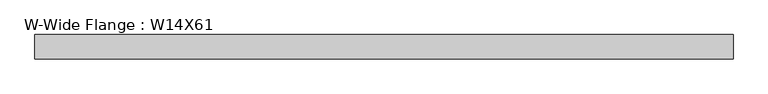
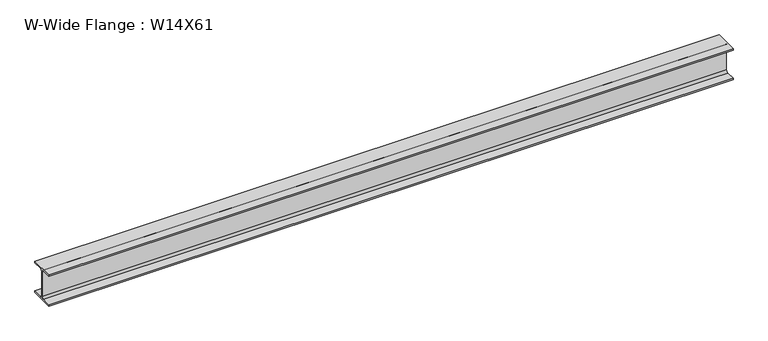
"""IFC4 building model written with IfcOpenShell, lengths in millimetres: beam geometry, W-Wide Flange : W14X61."""

import ifcopenshell
import ifcopenshell.guid

model = None  # the IFC model being written
_history = None  # IfcOwnerHistory: only IFC2X3 demands one
_inside = {}  # id of a spatial element -> (the spatial element, [elements in it])
_under = {}  # id of a project, library or spatial element -> (it, [spatial elements below it])
_declared = {}  # id of a project -> (the project, [libraries it declares])
_typed = {}  # id of a type object -> (the type object, [elements of that type])
_made_of = {}  # id of a material, layer set ... -> (it, [elements and type objects made of it])


def new_model(schema):
    """Start an empty IFC model of exactly this schema.

    Asked for "IFC4X3", IfcOpenShell would pick the latest addendum, in which some entities
    have other attributes; the version numbers below select the first issue.
    IFC2X3 requires an IfcOwnerHistory on every rooted entity: one is made here for all.
    """
    global model, _history
    if schema == "IFC4X3":
        model = ifcopenshell.file(schema_version=(4, 3, 0, 0))
    else:
        model = ifcopenshell.file(schema=schema)
    _inside.clear()
    _under.clear()
    _declared.clear()
    _typed.clear()
    _made_of.clear()
    _history = None
    if model.schema == "IFC2X3":
        org = make("IfcOrganization", Name="unknown")
        user = make(
            "IfcPersonAndOrganization",
            ThePerson=make("IfcPerson", FamilyName="unknown"),
            TheOrganization=org,
        )
        app = make(
            "IfcApplication",
            ApplicationDeveloper=org,
            Version="unknown",
            ApplicationFullName="unknown",
            ApplicationIdentifier="unknown",
        )
        _history = make(
            "IfcOwnerHistory",
            OwningUser=user,
            OwningApplication=app,
            ChangeAction="ADDED",
            CreationDate=0,
        )
    return model


def make(cls, **values):
    """One entity of the class cls with the attributes given. An attribute that is None is left unset."""
    return model.create_entity(
        cls, **{name: value for name, value in values.items() if value is not None}
    )


def rooted(cls, **values):
    """An entity with a GlobalId (a new one), such as an element, a storey or a relation."""
    return make(cls, GlobalId=ifcopenshell.guid.new(), OwnerHistory=_history, **values)


def si_unit(unit_type, name, prefix=None):
    """IfcSIUnit, for example si_unit("LENGTHUNIT", "METRE", prefix="MILLI")."""
    return make("IfcSIUnit", UnitType=unit_type, Prefix=prefix, Name=name)


def assignment(units):
    """IfcUnitAssignment: the units of a project."""
    return None if units is None else make("IfcUnitAssignment", Units=units)


def point(xyz):
    """IfcCartesianPoint."""
    return None if xyz is None else make("IfcCartesianPoint", Coordinates=xyz)


def direction(xyz):
    """IfcDirection."""
    return None if xyz is None else make("IfcDirection", DirectionRatios=xyz)


def frame(location, z_axis=None, x_axis=None):
    """IfcAxis2Placement3D, a coordinate frame: its origin and axes. An axis left out is left unset."""
    return make(
        "IfcAxis2Placement3D",
        Location=point(location),
        Axis=direction(z_axis),
        RefDirection=direction(x_axis),
    )


def frame_2d(location, x_axis=None):
    """IfcAxis2Placement2D, a coordinate frame in the plane: its origin and x axis."""
    return make(
        "IfcAxis2Placement2D", Location=point(location), RefDirection=direction(x_axis)
    )


def origin():
    """The frame at (0, 0, 0) with its axes left unset."""
    return frame((0.0, 0.0, 0.0))


def place(relative_to, where):
    """IfcLocalPlacement: puts the frame where relative to a parent placement (None: the world)."""
    return make(
        "IfcLocalPlacement", PlacementRelTo=relative_to, RelativePlacement=where
    )


def context(
    kind, dimensions, precision=None, world=None, true_north=None, identifier=None
):
    """IfcGeometricRepresentationContext, for example the 3D "Model" context."""
    return make(
        "IfcGeometricRepresentationContext",
        ContextIdentifier=identifier,
        ContextType=kind,
        CoordinateSpaceDimension=dimensions,
        Precision=precision,
        WorldCoordinateSystem=world,
        TrueNorth=true_north,
    )


def project(units=None, contexts=None):
    """IfcProject with its units and contexts."""
    return rooted(
        "IfcProject",
        Name="project",
        RepresentationContexts=contexts,
        UnitsInContext=assignment(units),
    )


def spatial(cls, under=None, at=None, **own):
    """A site, building, storey or space (cls), placed at a placement, below another one or the project."""
    s = rooted(cls, ObjectPlacement=at, **own)
    if under is not None:
        _under.setdefault(under.id(), (under, []))[1].append(s)
    return s


def polyline(points):
    """IfcPolyline through the points."""
    return make("IfcPolyline", Points=[point(p) for p in points])


def circle_curve(where, radius):
    """IfcCircle in the frame where."""
    return make("IfcCircle", Position=where, Radius=radius)


def trimmed(basis, trim1, trim2, sense, master):
    """IfcTrimmedCurve: the piece of a basis curve between two trims."""
    return make(
        "IfcTrimmedCurve",
        BasisCurve=basis,
        Trim1=trim1,
        Trim2=trim2,
        SenseAgreement=sense,
        MasterRepresentation=master,
    )


def segment(curve, same_sense, transition):
    """IfcCompositeCurveSegment."""
    return make(
        "IfcCompositeCurveSegment",
        Transition=transition,
        SameSense=same_sense,
        ParentCurve=curve,
    )


def composite_curve(segments, self_intersect=None):
    """IfcCompositeCurve: segments joined end to end."""
    return make("IfcCompositeCurve", Segments=segments, SelfIntersect=self_intersect)


def outline(outer, holes=None, kind="AREA"):
    """IfcArbitraryClosedProfileDef: a profile drawn as a closed curve; with holes, ...WithVoids."""
    if holes is None:
        return make("IfcArbitraryClosedProfileDef", ProfileType=kind, OuterCurve=outer)
    return make(
        "IfcArbitraryProfileDefWithVoids",
        ProfileType=kind,
        OuterCurve=outer,
        InnerCurves=holes,
    )


def extrude(swept, where, along, depth):
    """IfcExtrudedAreaSolid: the profile swept, set in the frame where, extruded along a direction by depth."""
    return make(
        "IfcExtrudedAreaSolid",
        SweptArea=swept,
        Position=where,
        ExtrudedDirection=direction(along),
        Depth=depth,
    )


def shape(context_of_items, identifier, shape_type, items):
    """IfcShapeRepresentation: the items that make up one representation, for example the "Body"."""
    return make(
        "IfcShapeRepresentation",
        ContextOfItems=context_of_items,
        RepresentationIdentifier=identifier,
        RepresentationType=shape_type,
        Items=items,
    )


def source(mapping_origin, context_of_items, identifier, shape_type, items):
    """IfcRepresentationMap: a shape defined once, which mapped items show again and again."""
    return make(
        "IfcRepresentationMap",
        MappingOrigin=mapping_origin,
        MappedRepresentation=shape(context_of_items, identifier, shape_type, items),
    )


def transform(
    local_origin,
    x_axis=None,
    y_axis=None,
    z_axis=None,
    scale=None,
    scale2=None,
    scale3=None,
    uniform=True,
):
    """IfcCartesianTransformationOperator3D, or its non-uniform kind. x_axis, y_axis, z_axis: its Axis1, 2, 3."""
    if uniform:
        return make(
            "IfcCartesianTransformationOperator3D",
            Axis1=direction(x_axis),
            Axis2=direction(y_axis),
            LocalOrigin=point(local_origin),
            Scale=scale,
            Axis3=direction(z_axis),
        )
    return make(
        "IfcCartesianTransformationOperator3DnonUniform",
        Axis1=direction(x_axis),
        Axis2=direction(y_axis),
        LocalOrigin=point(local_origin),
        Scale=scale,
        Axis3=direction(z_axis),
        Scale2=scale2,
        Scale3=scale3,
    )


def mapped(mapping_source, mapping_target):
    """IfcMappedItem: shows the shape of a source again, moved by a transform."""
    return make(
        "IfcMappedItem", MappingSource=mapping_source, MappingTarget=mapping_target
    )


def made_of(thing, what):
    """Note that an element or type object is made of a material, layer set ...; save() writes the relation."""
    if what is not None:
        _made_of.setdefault(what.id(), (what, []))[1].append(thing)
    return thing


def element(
    cls,
    number,
    at=None,
    inside=None,
    cuts=None,
    type_object=None,
    material=None,
    context=None,
    identifier="Body",
    shape_type=None,
    held_by="IfcProductDefinitionShape",
    body=None,
    shapes=None,
    **own,
):
    """One element of the class cls, such as IfcWall. Its Tag is "e" and its number.

    at: its placement. inside: the storey or other place that contains it. cuts: it is an
    opening in that element (IfcRelVoidsElement). A single representation is given by context,
    identifier, shape_type and body (its items); several are given by shapes. held_by: the class
    of the entity that holds the representations. save() writes the other relations.
    """
    e = rooted(cls, Tag="e%d" % number, ObjectPlacement=at, **own)
    if body is not None:
        shapes = [shape(context, identifier, shape_type, body)]
    if shapes is not None:
        e.Representation = make(held_by, Representations=shapes)
    if inside is not None:
        _inside.setdefault(inside.id(), (inside, []))[1].append(e)
    if cuts is not None:
        rooted(
            "IfcRelVoidsElement", RelatingBuildingElement=cuts, RelatedOpeningElement=e
        )
    if type_object is not None:
        _typed.setdefault(type_object.id(), (type_object, []))[1].append(e)
    return made_of(e, material)


def aggregate(whole, parts):
    """IfcRelAggregates: a whole, such as a stair, and the parts it consists of."""
    return rooted("IfcRelAggregates", RelatingObject=whole, RelatedObjects=parts)


def save(model, path):
    """Write the relations noted so far, then the file.

    IfcRelAggregates (storeys below a building ...), IfcRelContainedInSpatialStructure (elements
    in a storey), IfcRelDefinesByType, IfcRelAssociatesMaterial and IfcRelDeclares: one each for
    every whole, place, type object, material and project.
    """
    for whole, parts in _under.values():
        aggregate(whole, parts)
    for where, things in _inside.values():
        rooted(
            "IfcRelContainedInSpatialStructure",
            RelatedElements=things,
            RelatingStructure=where,
        )
    for kind, things in _typed.values():
        rooted("IfcRelDefinesByType", RelatedObjects=things, RelatingType=kind)
    for what, things in _made_of.values():
        rooted("IfcRelAssociatesMaterial", RelatedObjects=things, RelatingMaterial=what)
    for by, libraries in _declared.values():
        rooted("IfcRelDeclares", RelatingContext=by, RelatedDefinitions=libraries)
    model.write(path)


def w_wide_flange_w14x61_a1268b43(model_context):
    return source(origin(), model_context, "Body", "SweptSolid", [
        extrude(outline(composite_curve([segment(polyline([(127.0, -160.147), (127.0, -176.53), (-127.0, -176.53), (-127.0, -160.147), (-26.4795, -160.147)]), True, "CONTINUOUS"), segment(trimmed(circle_curve(frame_2d((-26.4795, -138.43)), 21.717), [point((-26.4795, -160.147))], [point((-4.7625, -138.43))], True, "CARTESIAN"), True, "CONTINUOUS"), segment(polyline([(-4.7625, -138.43), (-4.7625, 138.43)]), True, "CONTINUOUS"), segment(trimmed(circle_curve(frame_2d((-26.4795, 138.43)), 21.717), [point((-4.7625, 138.43))], [point((-26.4795, 160.147))], True, "CARTESIAN"), True, "CONTINUOUS"), segment(polyline([(-26.4795, 160.147), (-127.0, 160.147), (-127.0, 176.53), (127.0, 176.53), (127.0, 160.147), (26.4795, 160.147)]), True, "CONTINUOUS"), segment(trimmed(circle_curve(frame_2d((26.4795, 138.43)), 21.717), [point((26.4795, 160.147))], [point((4.7625, 138.43))], True, "CARTESIAN"), True, "CONTINUOUS"), segment(polyline([(4.7625, 138.43), (4.7625, -138.43)]), True, "CONTINUOUS"), segment(trimmed(circle_curve(frame_2d((26.4795, -138.43)), 21.717), [point((4.7625, -138.43))], [point((26.4795, -160.147))], True, "CARTESIAN"), True, "CONTINUOUS"), segment(polyline([(26.4795, -160.147), (127.0, -160.147)]), True, "CONTINUOUS")], self_intersect=False)), frame((-3645.6441406, 0.0, 0.0), z_axis=(1.0, 0.0, 0.0), x_axis=(0.0, 1.0, 0.0)), (0.0, 0.0, 1.0), 7291.2882813),
    ])


if __name__ == "__main__":
    model = new_model("IFC4")
    model_context = context("Model", 3, world=origin())
    ifc_project = project(units=[si_unit("LENGTHUNIT", "METRE", prefix="MILLI")], contexts=[model_context])
    site = spatial("IfcSite", under=ifc_project)
    building = spatial("IfcBuilding", under=site)
    placement = place(None, origin())
    w_wide_flange_w14x61_shape = w_wide_flange_w14x61_a1268b43(model_context)
    element("IfcBeam", 1, ObjectType="W-Wide Flange : W14X61", at=placement, inside=building, context=model_context, shape_type="MappedRepresentation", body=[
        mapped(w_wide_flange_w14x61_shape, transform((0.0, 0.0, 0.0), x_axis=(1.0, 0.0, 0.0), y_axis=(0.0, 1.0, 0.0), z_axis=(0.0, 0.0, 1.0))),
    ])
    save(model, "model.ifc")

# Revit data of these elements
# Type "W-Wide Flange : W14X61"
#   Assembly Code = "B10"
#   W = 61
#   Length [instance default] = 1524 mm
#   bf = 254 mm
#   d = 353.06 mm
#   k = 38.1 mm
#   k2 = 21.717 mm
#   tf = 16.383 mm
#   tw = 9.525 mm
#   A = 0.0115484 m²
#   Structural Material [instance default] = Steel ASTM A992
# Element 1 (IfcBeam, "W-Wide Flange : W14X61")
#   Structural Material = Aluminum, Anodized Red
#   Materials on its faces: "Aluminum, Anodized Red"
# Materials
#   "Steel ASTM A992": class "Metal", colour RGB 128 0 0, transparency 0, Description = "Structural steel 50ksi", Cost = 0
#   "Aluminum, Anodized Red": class "Metal", colour RGB 120 120 120, transparency 0, Description = "Anodized aluminum, red", Cost = 0
